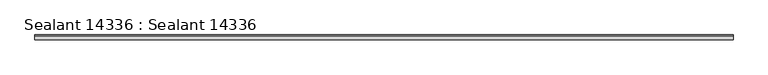
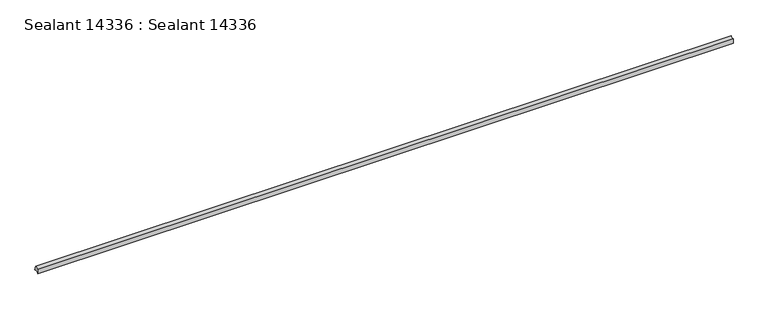
"""IFC4 building model written with IfcOpenShell, lengths in millimetres: proxy geometry, Sealant 14336 : Sealant 14336."""

from ifc_helpers import new_model, si_unit, point, frame, frame_2d, origin, place, context, project, spatial, polyline, circle_curve, trimmed, segment, composite_curve, outline, extrude, source, transform, mapped, element, save


def sealant_14336_sealant_14336_dc2ed740(model_context):
    return source(origin(), model_context, "Body", "SweptSolid", [
        extrude(outline(composite_curve([segment(polyline([(2285.7732111, 44328.9010742), (2290.0339532, 44315.1393555)]), True, "CONTINUOUS"), segment(trimmed(circle_curve(frame_2d((2284.6073494, 44305.9766143)), 10.6491246), [point((2290.0339532, 44315.1393555))], [point((2275.7760506, 44311.927414))], True, "CARTESIAN"), True, "CONTINUOUS"), segment(polyline([(2275.7760506, 44311.927414), (2275.7760506, 44325.8058705)]), True, "CONTINUOUS"), segment(trimmed(circle_curve(frame_2d((2278.2859341, 44335.3916832)), 9.9089516), [point((2275.7760506, 44325.8058705))], [point((2285.7732111, 44328.9010742))], True, "CARTESIAN"), True, "CONTINUOUS")], self_intersect=False)), frame((6470.1466437, 0.0, 0.0), z_axis=(1.0, 0.0, 0.0), x_axis=(0.0, 1.0, 0.0)), (0.0, 0.0, 1.0), 1999.85),
    ])


if __name__ == "__main__":
    model = new_model("IFC4")
    model_context = context("Model", 3, world=origin())
    ifc_project = project(units=[si_unit("LENGTHUNIT", "METRE", prefix="MILLI")], contexts=[model_context])
    site = spatial("IfcSite", under=ifc_project)
    building = spatial("IfcBuilding", under=site)
    placement = place(None, origin())
    sealant_14336_sealant_14336_shape = sealant_14336_sealant_14336_dc2ed740(model_context)
    element("IfcBuildingElementProxy", 1, Name="Sealant 14336 : Sealant 14336", ObjectType="Sealant 14336 : Sealant 14336", at=placement, inside=building, context=model_context, shape_type="MappedRepresentation", body=[
        mapped(sealant_14336_sealant_14336_shape, transform((0.0, 0.0, 0.0), x_axis=(1.0, 0.0, 0.0), y_axis=(0.0, 1.0, 0.0), z_axis=(0.0, 0.0, 1.0))),
    ])
    save(model, "model.ifc")

# Revit data of these elements
# Type "Sealant 14336 : Sealant 14336"
#   NameOverride = "Sealant"
# Element 1 (IfcBuildingElementProxy, "Sealant 14336 : Sealant 14336")
#   Materials on its faces: "SEALANT AND BACKER ROD WHERE NECESSARY"
# Materials
#   "SEALANT AND BACKER ROD WHERE NECESSARY": class "Unassigned", colour RGB 225 240 198, transparency 0, Cost = 0
